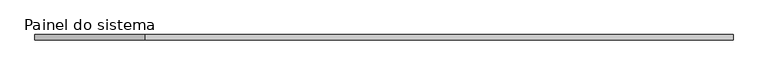
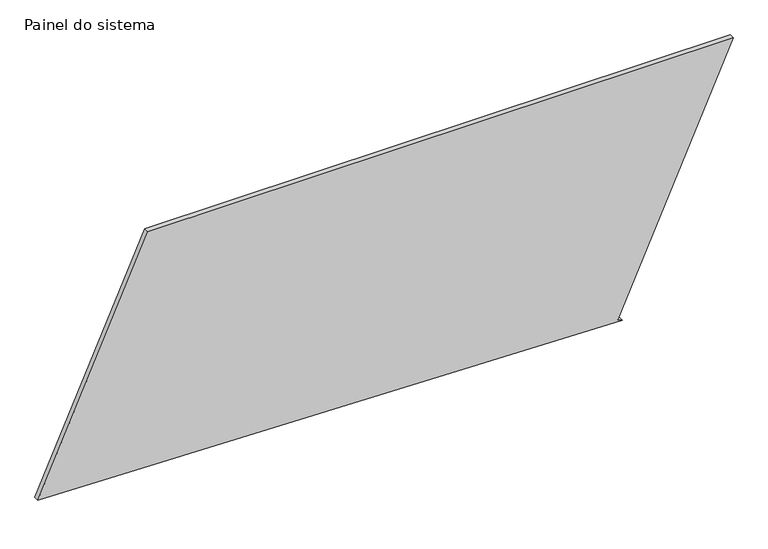
"""IFC4 building model written with IfcOpenShell, lengths in millimetres: plate geometry, Painel do sistema : Envidraçado."""

from ifc_helpers import new_model, si_unit, frame, origin, place, context, project, spatial, polyline, outline, extrude, source, transform, mapped, element, save


def painel_do_sistema_3832c5f9(model_context):
    return source(origin(), model_context, "Body", "SweptSolid", [
        extrude(outline(polyline([(0.0, 1130.4656126), (10.2299965, 1107.6544931), (1238.7565718, 1658.6060869), (1238.7565718, -1133.4850228), (67.8276013, -1658.6060869), (0.0, 1130.4656126)])), frame((0.0, 24.5, 0.0), z_axis=(0.0, 1.0, 0.0), x_axis=(0.0, 0.0, 1.0)), (0.0, 0.0, 1.0), 25.0),
    ])


if __name__ == "__main__":
    model = new_model("IFC4")
    model_context = context("Model", 3, world=origin())
    ifc_project = project(units=[si_unit("LENGTHUNIT", "METRE", prefix="MILLI")], contexts=[model_context])
    site = spatial("IfcSite", under=ifc_project)
    building = spatial("IfcBuilding", under=site)
    placement = place(None, origin())
    painel_do_sistema_shape = painel_do_sistema_3832c5f9(model_context)
    element("IfcPlate", 1, ObjectType="Painel do sistema : Envidraçado", at=placement, inside=building, context=model_context, shape_type="MappedRepresentation", body=[
        mapped(painel_do_sistema_shape, transform((0.0, 0.0, 0.0), x_axis=(1.0, 0.0, 0.0), y_axis=(0.0, 1.0, 0.0), z_axis=(0.0, 0.0, 1.0))),
    ])
    save(model, "model.ifc")

# Revit data of these elements
# Type "Painel do sistema : Envidraçado"
#   Construction Type Id = "GSP4R"
#   Analytic Construction = "Vidraça única Pilkington 1/8 pol"
#   Visual Light Transmittance = 0.9
#   Solar Heat Gain Coefficient = 0.86
#   Heat Transfer Coefficient (U) = 6.7069 W/(m²·K)
# Element 1 (IfcPlate, "Painel do sistema : Envidraçado")
#   Materials on its faces: "Vidro"
# Materials
#   "Vidro": class "Vidro", colour RGB 0 128 192, transparency 0.9, Description = "Vidro de sílica", Cost = 0
